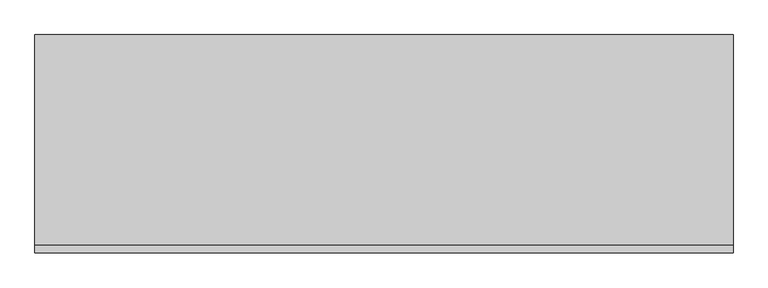
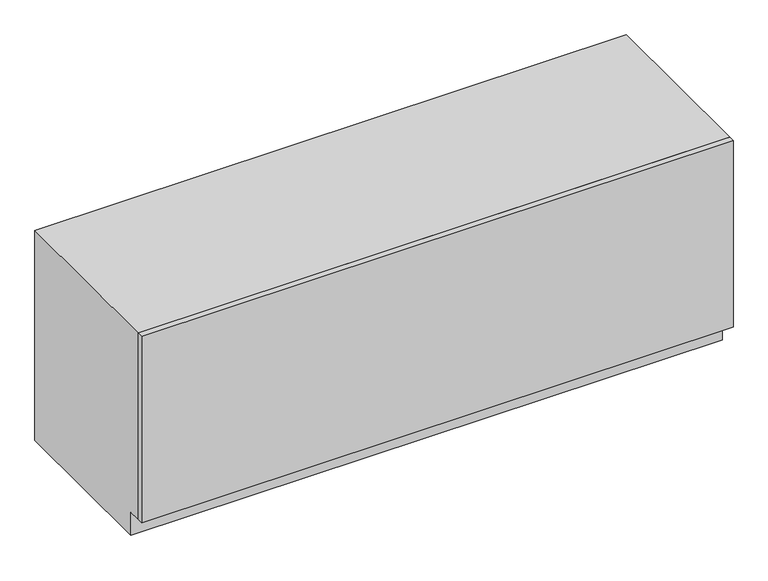
"""IFC4 building model written with IfcOpenShell, lengths in millimetres: furniture geometry, OD_CW_Base Cabinet : OD_CW_Base Cabinet."""

from ifc_helpers import new_model, si_unit, frame, origin, place, context, project, spatial, polyline, outline, extrude, source, transform, mapped, element, save


def furniture_8383f002(model_context):
    return source(origin(), model_context, "Body", "SweptSolid", [
        extrude(outline(polyline([(18.7377049, -127.0), (2457.1377049, -127.0), (2457.1377049, -152.4), (18.7377049, -152.4), (18.7377049, -127.0)])), frame((0.0, 0.0, 101.6), z_axis=(0.0, 0.0, 1.0), x_axis=(1.0, 0.0, 0.0)), (0.0, 0.0, 1.0), 812.8),
        extrude(outline(polyline([(-127.0, 914.4), (609.6, 914.4), (609.6, 0.0), (-76.2, 0.0), (-76.2, 101.6), (-127.0, 101.6), (-127.0, 914.4)])), frame((18.7377049, 0.0, 0.0), z_axis=(1.0, 0.0, 0.0), x_axis=(0.0, 1.0, 0.0)), (0.0, 0.0, 1.0), 2438.4),
    ])


if __name__ == "__main__":
    model = new_model("IFC4")
    model_context = context("Model", 3, world=origin())
    ifc_project = project(units=[si_unit("LENGTHUNIT", "METRE", prefix="MILLI")], contexts=[model_context])
    site = spatial("IfcSite", under=ifc_project)
    building = spatial("IfcBuilding", under=site)
    placement = place(None, origin())
    furniture_shape = furniture_8383f002(model_context)
    element("IfcFurniture", 1, ObjectType="OD_CW_Base Cabinet : OD_CW_Base Cabinet", at=placement, inside=building, context=model_context, shape_type="MappedRepresentation", body=[
        mapped(furniture_shape, transform((0.0, 0.0, 0.0), x_axis=(1.0, 0.0, 0.0), y_axis=(0.0, 1.0, 0.0), z_axis=(0.0, 0.0, 1.0))),
    ])
    save(model, "model.ifc")

# Revit data of these elements
# Type "OD_CW_Base Cabinet : OD_CW_Base Cabinet"
#   OD_CW_Width [instance default] = 2' - 10"
#   OD_CW_Length [instance default] = 8' - 0"
#   OD_CW_Height [instance default] = 2' - 3"
#   Depth = 2' - 0"
#   Height = 3' - 0"
#   Width = 4' - 0"
#   OD_CW_Material_Front Panel [instance default] = none
#   OD_CW_Material_Body [instance default] = none
# Element 1 (IfcFurniture, "OD_CW_Base Cabinet : OD_CW_Base Cabinet")
#   OD_CW_Width = 2' - 6"
#   OD_CW_Height = 3' - 0"
#   OD_CW_Material_Body = PREP TABLE WITH SINK
#   Materials on its faces: "PREP TABLE WITH SINK", "CASEWORK"
# Materials
#   "PREP TABLE WITH SINK": class "Generic", colour RGB 187 187 187, transparency 0, Cost = 0
#   "CASEWORK": class "Generic", colour RGB 181 181 181, transparency 0, Cost = 0
